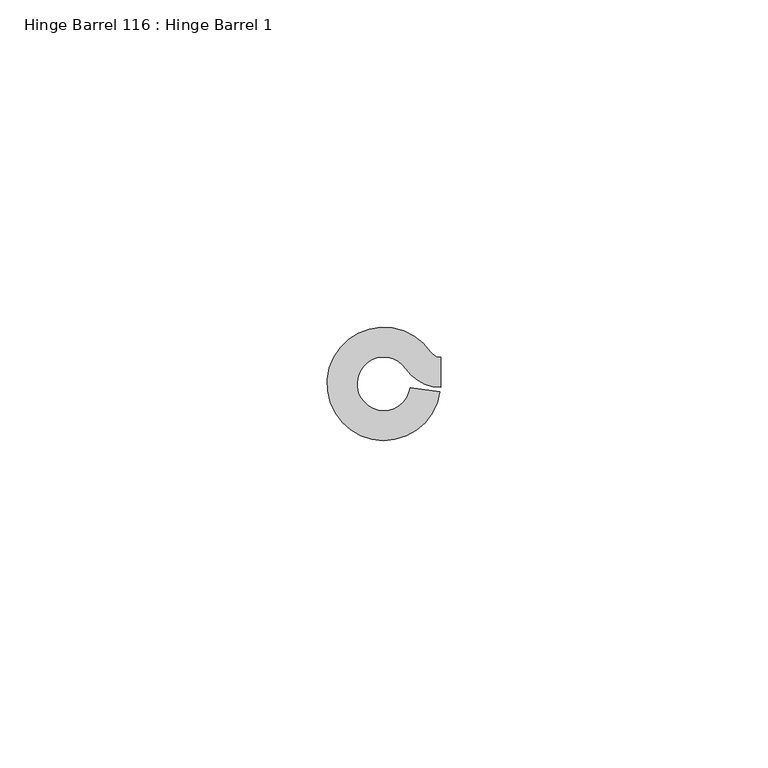
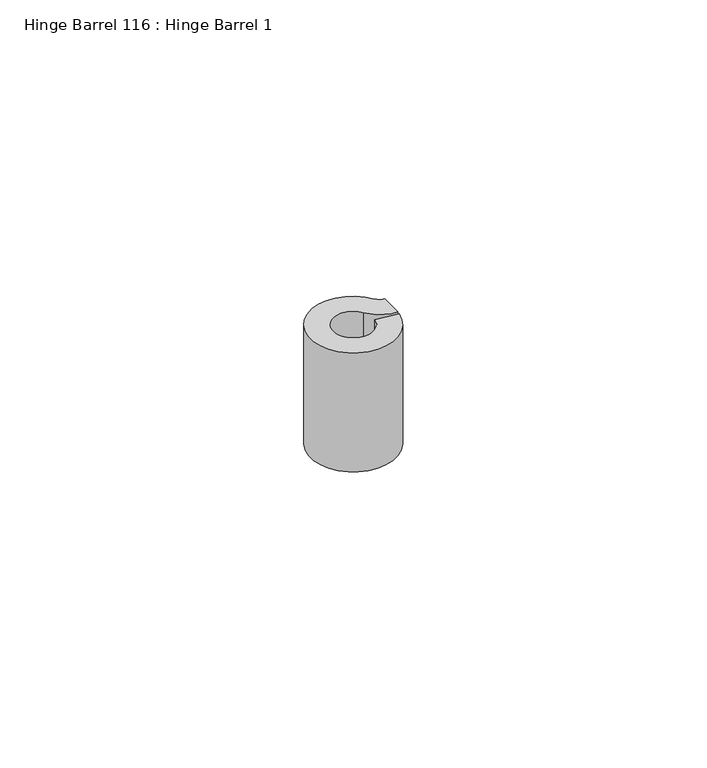
"""IFC4 building model written with IfcOpenShell, lengths in millimetres: proxy geometry, Hinge Barrel 116 : Hinge Barrel 1."""

from ifc_helpers import new_model, si_unit, point, frame, frame_2d, origin, place, context, project, spatial, polyline, circle_curve, trimmed, segment, composite_curve, outline, extrude, source, transform, mapped, element, save


def hinge_barrel_116_hinge_barrel_1_4b375d58(model_context):
    return source(origin(), model_context, "Body", "SweptSolid", [
        extrude(outline(composite_curve([segment(trimmed(circle_curve(frame_2d((587319.1320739, -534100.7049841)), 4.0894), [point((587322.5194669, -534098.4139665))], [point((587323.1821338, -534101.2708529))], True, "CARTESIAN"), True, "CONTINUOUS"), segment(polyline([(587323.1821338, -534101.2708529), (587327.7022899, -534101.9024028)]), True, "CONTINUOUS"), segment(trimmed(circle_curve(frame_2d((587319.1320739, -534100.7049841)), 8.6534625), [point((587327.7022899, -534101.9024028))], [point((587326.3000393, -534095.8570273))], False, "CARTESIAN"), True, "CONTINUOUS"), segment(trimmed(circle_curve(frame_2d((587327.8245257, -534094.8259615)), 1.8404226), [point((587326.3000393, -534095.8570273))], [point((587327.8245257, -534096.6663841))], True, "CARTESIAN"), True, "CONTINUOUS"), segment(polyline([(587327.8245257, -534096.6663841), (587327.8245257, -534101.2304466)]), True, "CONTINUOUS"), segment(trimmed(circle_curve(frame_2d((587327.8245257, -534094.8259615)), 6.4044851), [point((587327.8245257, -534101.2304466))], [point((587322.5194669, -534098.4139665))], False, "CARTESIAN"), True, "CONTINUOUS")], self_intersect=False)), frame((0.0, 0.0, 1962.15), z_axis=(0.0, 0.0, 1.0), x_axis=(1.0, 0.0, 0.0)), (0.0, 0.0, 1.0), 25.4),
    ])


if __name__ == "__main__":
    model = new_model("IFC4")
    model_context = context("Model", 3, world=origin())
    ifc_project = project(units=[si_unit("LENGTHUNIT", "METRE", prefix="MILLI")], contexts=[model_context])
    site = spatial("IfcSite", under=ifc_project)
    building = spatial("IfcBuilding", under=site)
    placement = place(None, origin())
    hinge_barrel_116_hinge_barrel_1_shape = hinge_barrel_116_hinge_barrel_1_4b375d58(model_context)
    element("IfcBuildingElementProxy", 1, Name="Hinge Barrel 116 : Hinge Barrel 1", ObjectType="Hinge Barrel 116 : Hinge Barrel 1", at=placement, inside=building, context=model_context, shape_type="MappedRepresentation", body=[
        mapped(hinge_barrel_116_hinge_barrel_1_shape, transform((0.0, 0.0, 0.0), x_axis=(1.0, 0.0, 0.0), y_axis=(0.0, 1.0, 0.0), z_axis=(0.0, 0.0, 1.0))),
    ])
    save(model, "model.ifc")

# Revit data of these elements
# Element 1 (IfcBuildingElementProxy, "Hinge Barrel 116 : Hinge Barrel 1")
#   Materials on its faces: "6\"X6\" WELD-ON STL BUTT HINGE"
# Materials
#   "6\"X6\" WELD-ON STL BUTT HINGE": class "Metal", colour RGB 189 187 185, transparency 0, Description = "Carbon steel", Cost = 0
